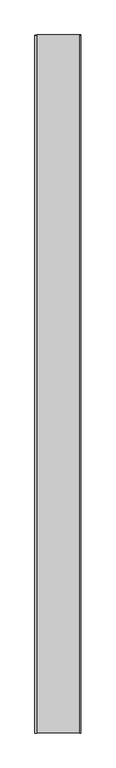
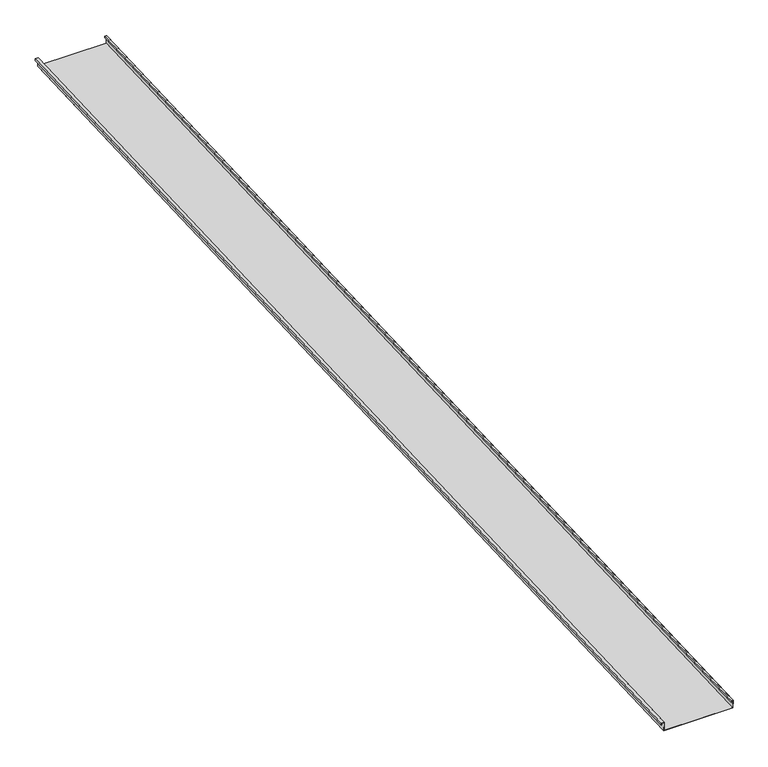
"""IFC4 building model written with IfcOpenShell, lengths in millimetres: proxy geometry, Generic Models 2:Generic Models 2:310765:Generic Models 2:310765 : Generic Models 2:Generic Models 2:310765:129 : Generic Models 2:Generic Models 2:310765:Generic Models 2:310765 : Generic Models 2:Generic Models 2:310765:300385."""

from ifc_helpers import new_model, si_unit, frame, origin, place, context, project, spatial, polyline, outline, extrude, source, transform, mapped, element, save


def generic_models_e1e9d50f(model_context):
    return source(origin(), model_context, "Body", "SweptSolid", [
        extrude(outline(polyline([(1.5875, 0.0), (1.5875, 50.8), (407.9875, 50.8), (407.9875, 1.5875), (396.875, 1.5875), (396.875, 11.1125), (398.4625, 11.1125), (398.4625, 3.175), (406.4, 3.175), (406.4, 49.2125), (3.175, 49.2125), (3.175, -1.5874999), (-14.2875, -1.5874999), (-14.2875, 9.525), (-12.7, 9.525), (-12.7, 0.0), (1.5875, 0.0)])), frame((660124.4263072, -581354.4345603, 3902.6697972), z_axis=(0.0, 0.9991330730923568, 0.041630544712067834), x_axis=(1.0, 0.0, 0.0)), (0.0, 0.0, 1.0), 6400.8),
    ])


if __name__ == "__main__":
    model = new_model("IFC4")
    model_context = context("Model", 3, world=origin())
    ifc_project = project(units=[si_unit("LENGTHUNIT", "METRE", prefix="MILLI")], contexts=[model_context])
    site = spatial("IfcSite", under=ifc_project)
    building = spatial("IfcBuilding", under=site)
    placement = place(None, origin())
    generic_models_shape = generic_models_e1e9d50f(model_context)
    element("IfcBuildingElementProxy", 1, Name="Generic Models 2:Generic Models 2:310765:Generic Models 2:310765 : Generic Models 2:Generic Models 2:310765:129 : Generic Models 2:Generic Models 2:310765:Generic Models 2:310765 : Generic Models 2:Generic Models 2:310765:300385", ObjectType="Generic Models 2:Generic Models 2:310765:Generic Models 2:310765 : Generic Models 2:Generic Models 2:310765:129 : Generic Models 2:Generic Models 2:310765:Generic Models 2:310765 : Generic Models 2:Generic Models 2:310765:300385", at=placement, inside=building, context=model_context, shape_type="MappedRepresentation", body=[
        mapped(generic_models_shape, transform((0.0, 0.0, 0.0), x_axis=(1.0, 0.0, 0.0), y_axis=(0.0, 1.0, 0.0), z_axis=(0.0, 0.0, 1.0))),
    ])
    save(model, "model.ifc")

# Revit data of these elements
# Type "Generic Models 2:Generic Models 2:310765:Generic Models 2:310765 : Generic Models 2:Generic Models 2:310765:129 : Generic Models 2:Generic Models 2:310765:Generic Models 2:310765 : Generic Models 2:Generic Models 2:310765:300385"
#   NameOverride = "Generic Models 2:Generic Models 2:310765:Generic Models 2:310765 : Generic Models 2:Generic Models 2:310765:300385"
#   ObjectTypeOverride = "Generic Models 2:310765 : Generic Models 2:Generic Models 2:310765"
#   Reference = "Generic Models 2"
#   Tag = "300385"
# Element 1 (IfcBuildingElementProxy, "Generic Models 2:Generic Models 2:310765:Generic Models 2:310765 : Generic Models 2:Generic Models 2:310765:129 : Generic Models 2:Generic Models 2:310765:Generic Models 2:310765 : Generic Models 2:Generic Models 2:310765:300385")
#   Materials on its faces: "THERMAL BROKEN ALUMINUM STOREFRONT FOR POLYCARBONATE"
# Materials
#   "THERMAL BROKEN ALUMINUM STOREFRONT FOR POLYCARBONATE": class "Unassigned", colour RGB 244 244 244, transparency 0, Keynote = "M07611300.01", Cost = 0
